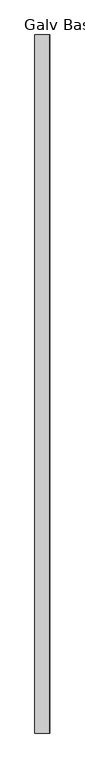
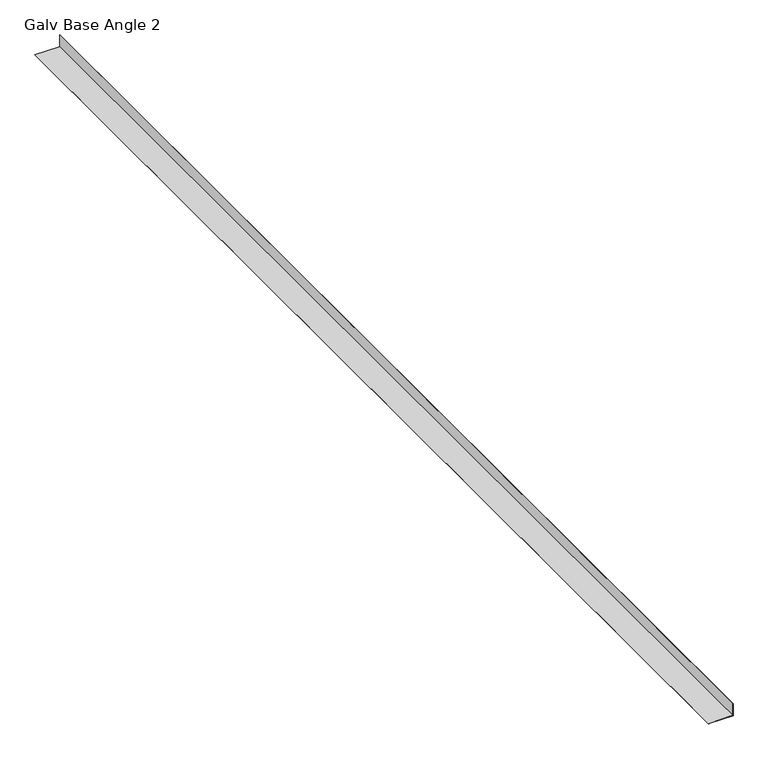
"""IFC4 building model written with IfcOpenShell, lengths in millimetres: proxy geometry, Galv Base Angle 2 : CF Galv L 4x2x16ga."""

import ifcopenshell
import ifcopenshell.guid

model = None  # the IFC model being written
_history = None  # IfcOwnerHistory: only IFC2X3 demands one
_inside = {}  # id of a spatial element -> (the spatial element, [elements in it])
_under = {}  # id of a project, library or spatial element -> (it, [spatial elements below it])
_declared = {}  # id of a project -> (the project, [libraries it declares])
_typed = {}  # id of a type object -> (the type object, [elements of that type])
_made_of = {}  # id of a material, layer set ... -> (it, [elements and type objects made of it])


def new_model(schema):
    """Start an empty IFC model of exactly this schema.

    Asked for "IFC4X3", IfcOpenShell would pick the latest addendum, in which some entities
    have other attributes; the version numbers below select the first issue.
    IFC2X3 requires an IfcOwnerHistory on every rooted entity: one is made here for all.
    """
    global model, _history
    if schema == "IFC4X3":
        model = ifcopenshell.file(schema_version=(4, 3, 0, 0))
    else:
        model = ifcopenshell.file(schema=schema)
    _inside.clear()
    _under.clear()
    _declared.clear()
    _typed.clear()
    _made_of.clear()
    _history = None
    if model.schema == "IFC2X3":
        org = make("IfcOrganization", Name="unknown")
        user = make(
            "IfcPersonAndOrganization",
            ThePerson=make("IfcPerson", FamilyName="unknown"),
            TheOrganization=org,
        )
        app = make(
            "IfcApplication",
            ApplicationDeveloper=org,
            Version="unknown",
            ApplicationFullName="unknown",
            ApplicationIdentifier="unknown",
        )
        _history = make(
            "IfcOwnerHistory",
            OwningUser=user,
            OwningApplication=app,
            ChangeAction="ADDED",
            CreationDate=0,
        )
    return model


def make(cls, **values):
    """One entity of the class cls with the attributes given. An attribute that is None is left unset."""
    return model.create_entity(
        cls, **{name: value for name, value in values.items() if value is not None}
    )


def rooted(cls, **values):
    """An entity with a GlobalId (a new one), such as an element, a storey or a relation."""
    return make(cls, GlobalId=ifcopenshell.guid.new(), OwnerHistory=_history, **values)


def si_unit(unit_type, name, prefix=None):
    """IfcSIUnit, for example si_unit("LENGTHUNIT", "METRE", prefix="MILLI")."""
    return make("IfcSIUnit", UnitType=unit_type, Prefix=prefix, Name=name)


def assignment(units):
    """IfcUnitAssignment: the units of a project."""
    return None if units is None else make("IfcUnitAssignment", Units=units)


def point(xyz):
    """IfcCartesianPoint."""
    return None if xyz is None else make("IfcCartesianPoint", Coordinates=xyz)


def direction(xyz):
    """IfcDirection."""
    return None if xyz is None else make("IfcDirection", DirectionRatios=xyz)


def frame(location, z_axis=None, x_axis=None):
    """IfcAxis2Placement3D, a coordinate frame: its origin and axes. An axis left out is left unset."""
    return make(
        "IfcAxis2Placement3D",
        Location=point(location),
        Axis=direction(z_axis),
        RefDirection=direction(x_axis),
    )


def origin():
    """The frame at (0, 0, 0) with its axes left unset."""
    return frame((0.0, 0.0, 0.0))


def place(relative_to, where):
    """IfcLocalPlacement: puts the frame where relative to a parent placement (None: the world)."""
    return make(
        "IfcLocalPlacement", PlacementRelTo=relative_to, RelativePlacement=where
    )


def context(
    kind, dimensions, precision=None, world=None, true_north=None, identifier=None
):
    """IfcGeometricRepresentationContext, for example the 3D "Model" context."""
    return make(
        "IfcGeometricRepresentationContext",
        ContextIdentifier=identifier,
        ContextType=kind,
        CoordinateSpaceDimension=dimensions,
        Precision=precision,
        WorldCoordinateSystem=world,
        TrueNorth=true_north,
    )


def project(units=None, contexts=None):
    """IfcProject with its units and contexts."""
    return rooted(
        "IfcProject",
        Name="project",
        RepresentationContexts=contexts,
        UnitsInContext=assignment(units),
    )


def spatial(cls, under=None, at=None, **own):
    """A site, building, storey or space (cls), placed at a placement, below another one or the project."""
    s = rooted(cls, ObjectPlacement=at, **own)
    if under is not None:
        _under.setdefault(under.id(), (under, []))[1].append(s)
    return s


def polyline(points):
    """IfcPolyline through the points."""
    return make("IfcPolyline", Points=[point(p) for p in points])


def outline(outer, holes=None, kind="AREA"):
    """IfcArbitraryClosedProfileDef: a profile drawn as a closed curve; with holes, ...WithVoids."""
    if holes is None:
        return make("IfcArbitraryClosedProfileDef", ProfileType=kind, OuterCurve=outer)
    return make(
        "IfcArbitraryProfileDefWithVoids",
        ProfileType=kind,
        OuterCurve=outer,
        InnerCurves=holes,
    )


def extrude(swept, where, along, depth):
    """IfcExtrudedAreaSolid: the profile swept, set in the frame where, extruded along a direction by depth."""
    return make(
        "IfcExtrudedAreaSolid",
        SweptArea=swept,
        Position=where,
        ExtrudedDirection=direction(along),
        Depth=depth,
    )


def shape(context_of_items, identifier, shape_type, items):
    """IfcShapeRepresentation: the items that make up one representation, for example the "Body"."""
    return make(
        "IfcShapeRepresentation",
        ContextOfItems=context_of_items,
        RepresentationIdentifier=identifier,
        RepresentationType=shape_type,
        Items=items,
    )


def source(mapping_origin, context_of_items, identifier, shape_type, items):
    """IfcRepresentationMap: a shape defined once, which mapped items show again and again."""
    return make(
        "IfcRepresentationMap",
        MappingOrigin=mapping_origin,
        MappedRepresentation=shape(context_of_items, identifier, shape_type, items),
    )


def transform(
    local_origin,
    x_axis=None,
    y_axis=None,
    z_axis=None,
    scale=None,
    scale2=None,
    scale3=None,
    uniform=True,
):
    """IfcCartesianTransformationOperator3D, or its non-uniform kind. x_axis, y_axis, z_axis: its Axis1, 2, 3."""
    if uniform:
        return make(
            "IfcCartesianTransformationOperator3D",
            Axis1=direction(x_axis),
            Axis2=direction(y_axis),
            LocalOrigin=point(local_origin),
            Scale=scale,
            Axis3=direction(z_axis),
        )
    return make(
        "IfcCartesianTransformationOperator3DnonUniform",
        Axis1=direction(x_axis),
        Axis2=direction(y_axis),
        LocalOrigin=point(local_origin),
        Scale=scale,
        Axis3=direction(z_axis),
        Scale2=scale2,
        Scale3=scale3,
    )


def mapped(mapping_source, mapping_target):
    """IfcMappedItem: shows the shape of a source again, moved by a transform."""
    return make(
        "IfcMappedItem", MappingSource=mapping_source, MappingTarget=mapping_target
    )


def made_of(thing, what):
    """Note that an element or type object is made of a material, layer set ...; save() writes the relation."""
    if what is not None:
        _made_of.setdefault(what.id(), (what, []))[1].append(thing)
    return thing


def element(
    cls,
    number,
    at=None,
    inside=None,
    cuts=None,
    type_object=None,
    material=None,
    context=None,
    identifier="Body",
    shape_type=None,
    held_by="IfcProductDefinitionShape",
    body=None,
    shapes=None,
    **own,
):
    """One element of the class cls, such as IfcWall. Its Tag is "e" and its number.

    at: its placement. inside: the storey or other place that contains it. cuts: it is an
    opening in that element (IfcRelVoidsElement). A single representation is given by context,
    identifier, shape_type and body (its items); several are given by shapes. held_by: the class
    of the entity that holds the representations. save() writes the other relations.
    """
    e = rooted(cls, Tag="e%d" % number, ObjectPlacement=at, **own)
    if body is not None:
        shapes = [shape(context, identifier, shape_type, body)]
    if shapes is not None:
        e.Representation = make(held_by, Representations=shapes)
    if inside is not None:
        _inside.setdefault(inside.id(), (inside, []))[1].append(e)
    if cuts is not None:
        rooted(
            "IfcRelVoidsElement", RelatingBuildingElement=cuts, RelatedOpeningElement=e
        )
    if type_object is not None:
        _typed.setdefault(type_object.id(), (type_object, []))[1].append(e)
    return made_of(e, material)


def aggregate(whole, parts):
    """IfcRelAggregates: a whole, such as a stair, and the parts it consists of."""
    return rooted("IfcRelAggregates", RelatingObject=whole, RelatedObjects=parts)


def save(model, path):
    """Write the relations noted so far, then the file.

    IfcRelAggregates (storeys below a building ...), IfcRelContainedInSpatialStructure (elements
    in a storey), IfcRelDefinesByType, IfcRelAssociatesMaterial and IfcRelDeclares: one each for
    every whole, place, type object, material and project.
    """
    for whole, parts in _under.values():
        aggregate(whole, parts)
    for where, things in _inside.values():
        rooted(
            "IfcRelContainedInSpatialStructure",
            RelatedElements=things,
            RelatingStructure=where,
        )
    for kind, things in _typed.values():
        rooted("IfcRelDefinesByType", RelatedObjects=things, RelatingType=kind)
    for what, things in _made_of.values():
        rooted("IfcRelAssociatesMaterial", RelatedObjects=things, RelatingMaterial=what)
    for by, libraries in _declared.values():
        rooted("IfcRelDeclares", RelatingContext=by, RelatedDefinitions=libraries)
    model.write(path)


def galv_base_angle_2_de8a329e(model_context):
    return source(origin(), model_context, "Body", "SweptSolid", [
        extrude(outline(polyline([(0.93726, 590250.3936739), (0.0, 590250.3936739), (0.0, 590351.9936739), (50.8, 590351.9936739), (50.8, 590351.0564139), (0.93726, 590351.0564139), (0.93726, 590250.3936739)])), frame((0.0, -536417.5913841, 0.0), z_axis=(0.0, 1.0, 0.0), x_axis=(0.0, 0.0, 1.0)), (0.0, 0.0, 1.0), 4743.45),
    ])


if __name__ == "__main__":
    model = new_model("IFC4")
    model_context = context("Model", 3, world=origin())
    ifc_project = project(units=[si_unit("LENGTHUNIT", "METRE", prefix="MILLI")], contexts=[model_context])
    site = spatial("IfcSite", under=ifc_project)
    building = spatial("IfcBuilding", under=site)
    placement = place(None, origin())
    galv_base_angle_2_shape = galv_base_angle_2_de8a329e(model_context)
    element("IfcBuildingElementProxy", 1, Name="Galv Base Angle 2 : CF Galv L 4x2x16ga", ObjectType="Galv Base Angle 2 : CF Galv L 4x2x16ga", at=placement, inside=building, context=model_context, shape_type="MappedRepresentation", body=[
        mapped(galv_base_angle_2_shape, transform((0.0, 0.0, 0.0), x_axis=(1.0, 0.0, 0.0), y_axis=(0.0, 1.0, 0.0), z_axis=(0.0, 0.0, 1.0))),
    ])
    save(model, "model.ifc")

# Revit data of these elements
# Element 1 (IfcBuildingElementProxy, "Galv Base Angle 2 : CF Galv L 4x2x16ga")
#   Materials on its faces: "4\"X2\" L - COLD-FORMED GALV."
# Materials
#   "4\"X2\" L - COLD-FORMED GALV.": class "Generic", colour RGB 143 142 141, transparency 0, Cost = 0
